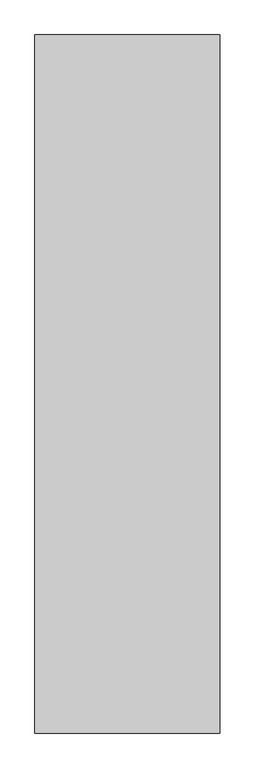
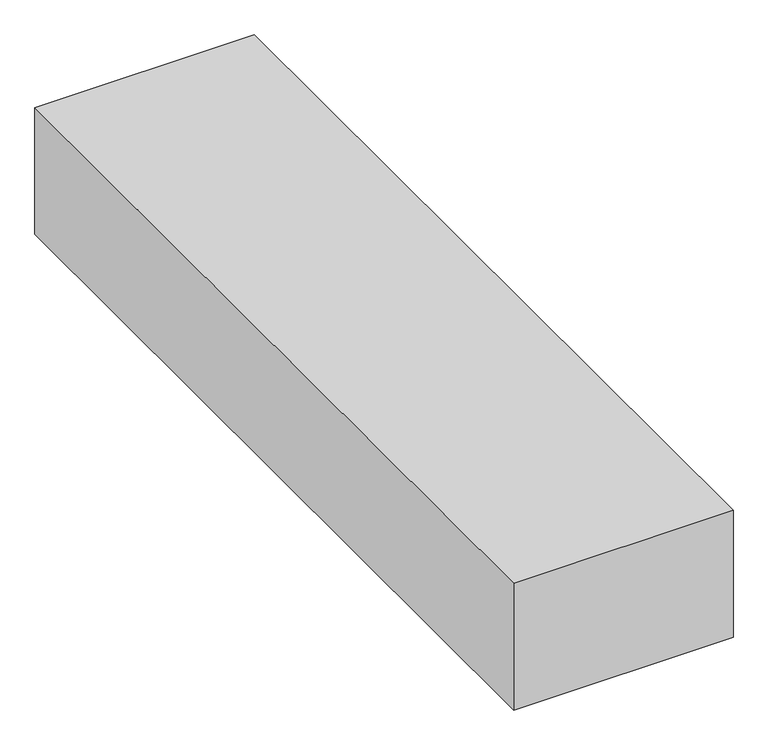
"""IFC4 building model written with IfcOpenShell, lengths in millimetres: proxy geometry, Space Planning Box_hec : Space Planning Box_hec."""

import ifcopenshell
import ifcopenshell.guid

model = None  # the IFC model being written
_history = None  # IfcOwnerHistory: only IFC2X3 demands one
_inside = {}  # id of a spatial element -> (the spatial element, [elements in it])
_under = {}  # id of a project, library or spatial element -> (it, [spatial elements below it])
_declared = {}  # id of a project -> (the project, [libraries it declares])
_typed = {}  # id of a type object -> (the type object, [elements of that type])
_made_of = {}  # id of a material, layer set ... -> (it, [elements and type objects made of it])


def new_model(schema):
    """Start an empty IFC model of exactly this schema.

    Asked for "IFC4X3", IfcOpenShell would pick the latest addendum, in which some entities
    have other attributes; the version numbers below select the first issue.
    IFC2X3 requires an IfcOwnerHistory on every rooted entity: one is made here for all.
    """
    global model, _history
    if schema == "IFC4X3":
        model = ifcopenshell.file(schema_version=(4, 3, 0, 0))
    else:
        model = ifcopenshell.file(schema=schema)
    _inside.clear()
    _under.clear()
    _declared.clear()
    _typed.clear()
    _made_of.clear()
    _history = None
    if model.schema == "IFC2X3":
        org = make("IfcOrganization", Name="unknown")
        user = make(
            "IfcPersonAndOrganization",
            ThePerson=make("IfcPerson", FamilyName="unknown"),
            TheOrganization=org,
        )
        app = make(
            "IfcApplication",
            ApplicationDeveloper=org,
            Version="unknown",
            ApplicationFullName="unknown",
            ApplicationIdentifier="unknown",
        )
        _history = make(
            "IfcOwnerHistory",
            OwningUser=user,
            OwningApplication=app,
            ChangeAction="ADDED",
            CreationDate=0,
        )
    return model


def make(cls, **values):
    """One entity of the class cls with the attributes given. An attribute that is None is left unset."""
    return model.create_entity(
        cls, **{name: value for name, value in values.items() if value is not None}
    )


def rooted(cls, **values):
    """An entity with a GlobalId (a new one), such as an element, a storey or a relation."""
    return make(cls, GlobalId=ifcopenshell.guid.new(), OwnerHistory=_history, **values)


def si_unit(unit_type, name, prefix=None):
    """IfcSIUnit, for example si_unit("LENGTHUNIT", "METRE", prefix="MILLI")."""
    return make("IfcSIUnit", UnitType=unit_type, Prefix=prefix, Name=name)


def assignment(units):
    """IfcUnitAssignment: the units of a project."""
    return None if units is None else make("IfcUnitAssignment", Units=units)


def point(xyz):
    """IfcCartesianPoint."""
    return None if xyz is None else make("IfcCartesianPoint", Coordinates=xyz)


def direction(xyz):
    """IfcDirection."""
    return None if xyz is None else make("IfcDirection", DirectionRatios=xyz)


def frame(location, z_axis=None, x_axis=None):
    """IfcAxis2Placement3D, a coordinate frame: its origin and axes. An axis left out is left unset."""
    return make(
        "IfcAxis2Placement3D",
        Location=point(location),
        Axis=direction(z_axis),
        RefDirection=direction(x_axis),
    )


def origin():
    """The frame at (0, 0, 0) with its axes left unset."""
    return frame((0.0, 0.0, 0.0))


def origin_with_axes():
    """The frame at (0, 0, 0) with the z axis (0, 0, 1) and the x axis (1, 0, 0) written out."""
    return frame((0.0, 0.0, 0.0), z_axis=(0.0, 0.0, 1.0), x_axis=(1.0, 0.0, 0.0))


def place(relative_to, where):
    """IfcLocalPlacement: puts the frame where relative to a parent placement (None: the world)."""
    return make(
        "IfcLocalPlacement", PlacementRelTo=relative_to, RelativePlacement=where
    )


def context(
    kind, dimensions, precision=None, world=None, true_north=None, identifier=None
):
    """IfcGeometricRepresentationContext, for example the 3D "Model" context."""
    return make(
        "IfcGeometricRepresentationContext",
        ContextIdentifier=identifier,
        ContextType=kind,
        CoordinateSpaceDimension=dimensions,
        Precision=precision,
        WorldCoordinateSystem=world,
        TrueNorth=true_north,
    )


def project(units=None, contexts=None):
    """IfcProject with its units and contexts."""
    return rooted(
        "IfcProject",
        Name="project",
        RepresentationContexts=contexts,
        UnitsInContext=assignment(units),
    )


def spatial(cls, under=None, at=None, **own):
    """A site, building, storey or space (cls), placed at a placement, below another one or the project."""
    s = rooted(cls, ObjectPlacement=at, **own)
    if under is not None:
        _under.setdefault(under.id(), (under, []))[1].append(s)
    return s


def polyline(points):
    """IfcPolyline through the points."""
    return make("IfcPolyline", Points=[point(p) for p in points])


def outline(outer, holes=None, kind="AREA"):
    """IfcArbitraryClosedProfileDef: a profile drawn as a closed curve; with holes, ...WithVoids."""
    if holes is None:
        return make("IfcArbitraryClosedProfileDef", ProfileType=kind, OuterCurve=outer)
    return make(
        "IfcArbitraryProfileDefWithVoids",
        ProfileType=kind,
        OuterCurve=outer,
        InnerCurves=holes,
    )


def extrude(swept, where, along, depth):
    """IfcExtrudedAreaSolid: the profile swept, set in the frame where, extruded along a direction by depth."""
    return make(
        "IfcExtrudedAreaSolid",
        SweptArea=swept,
        Position=where,
        ExtrudedDirection=direction(along),
        Depth=depth,
    )


def shape(context_of_items, identifier, shape_type, items):
    """IfcShapeRepresentation: the items that make up one representation, for example the "Body"."""
    return make(
        "IfcShapeRepresentation",
        ContextOfItems=context_of_items,
        RepresentationIdentifier=identifier,
        RepresentationType=shape_type,
        Items=items,
    )


def source(mapping_origin, context_of_items, identifier, shape_type, items):
    """IfcRepresentationMap: a shape defined once, which mapped items show again and again."""
    return make(
        "IfcRepresentationMap",
        MappingOrigin=mapping_origin,
        MappedRepresentation=shape(context_of_items, identifier, shape_type, items),
    )


def transform(
    local_origin,
    x_axis=None,
    y_axis=None,
    z_axis=None,
    scale=None,
    scale2=None,
    scale3=None,
    uniform=True,
):
    """IfcCartesianTransformationOperator3D, or its non-uniform kind. x_axis, y_axis, z_axis: its Axis1, 2, 3."""
    if uniform:
        return make(
            "IfcCartesianTransformationOperator3D",
            Axis1=direction(x_axis),
            Axis2=direction(y_axis),
            LocalOrigin=point(local_origin),
            Scale=scale,
            Axis3=direction(z_axis),
        )
    return make(
        "IfcCartesianTransformationOperator3DnonUniform",
        Axis1=direction(x_axis),
        Axis2=direction(y_axis),
        LocalOrigin=point(local_origin),
        Scale=scale,
        Axis3=direction(z_axis),
        Scale2=scale2,
        Scale3=scale3,
    )


def mapped(mapping_source, mapping_target):
    """IfcMappedItem: shows the shape of a source again, moved by a transform."""
    return make(
        "IfcMappedItem", MappingSource=mapping_source, MappingTarget=mapping_target
    )


def made_of(thing, what):
    """Note that an element or type object is made of a material, layer set ...; save() writes the relation."""
    if what is not None:
        _made_of.setdefault(what.id(), (what, []))[1].append(thing)
    return thing


def element(
    cls,
    number,
    at=None,
    inside=None,
    cuts=None,
    type_object=None,
    material=None,
    context=None,
    identifier="Body",
    shape_type=None,
    held_by="IfcProductDefinitionShape",
    body=None,
    shapes=None,
    **own,
):
    """One element of the class cls, such as IfcWall. Its Tag is "e" and its number.

    at: its placement. inside: the storey or other place that contains it. cuts: it is an
    opening in that element (IfcRelVoidsElement). A single representation is given by context,
    identifier, shape_type and body (its items); several are given by shapes. held_by: the class
    of the entity that holds the representations. save() writes the other relations.
    """
    e = rooted(cls, Tag="e%d" % number, ObjectPlacement=at, **own)
    if body is not None:
        shapes = [shape(context, identifier, shape_type, body)]
    if shapes is not None:
        e.Representation = make(held_by, Representations=shapes)
    if inside is not None:
        _inside.setdefault(inside.id(), (inside, []))[1].append(e)
    if cuts is not None:
        rooted(
            "IfcRelVoidsElement", RelatingBuildingElement=cuts, RelatedOpeningElement=e
        )
    if type_object is not None:
        _typed.setdefault(type_object.id(), (type_object, []))[1].append(e)
    return made_of(e, material)


def aggregate(whole, parts):
    """IfcRelAggregates: a whole, such as a stair, and the parts it consists of."""
    return rooted("IfcRelAggregates", RelatingObject=whole, RelatedObjects=parts)


def save(model, path):
    """Write the relations noted so far, then the file.

    IfcRelAggregates (storeys below a building ...), IfcRelContainedInSpatialStructure (elements
    in a storey), IfcRelDefinesByType, IfcRelAssociatesMaterial and IfcRelDeclares: one each for
    every whole, place, type object, material and project.
    """
    for whole, parts in _under.values():
        aggregate(whole, parts)
    for where, things in _inside.values():
        rooted(
            "IfcRelContainedInSpatialStructure",
            RelatedElements=things,
            RelatingStructure=where,
        )
    for kind, things in _typed.values():
        rooted("IfcRelDefinesByType", RelatedObjects=things, RelatingType=kind)
    for what, things in _made_of.values():
        rooted("IfcRelAssociatesMaterial", RelatedObjects=things, RelatingMaterial=what)
    for by, libraries in _declared.values():
        rooted("IfcRelDeclares", RelatingContext=by, RelatedDefinitions=libraries)
    model.write(path)


def generic_models_8b5775ea(model_context):
    return source(origin(), model_context, "Body", "SweptSolid", [
        extrude(outline(polyline([(4500.0, 17000.0), (4500.0, -17000.0), (-4500.0, -17000.0), (-4500.0, 17000.0), (4500.0, 17000.0)])), origin_with_axes(), (0.0, 0.0, 1.0), 5500.0),
    ])


if __name__ == "__main__":
    model = new_model("IFC4")
    model_context = context("Model", 3, world=origin())
    ifc_project = project(units=[si_unit("LENGTHUNIT", "METRE", prefix="MILLI")], contexts=[model_context])
    site = spatial("IfcSite", under=ifc_project)
    building = spatial("IfcBuilding", under=site)
    placement = place(None, origin())
    generic_models_shape = generic_models_8b5775ea(model_context)
    element("IfcBuildingElementProxy", 1, Name="Space Planning Box_hec : Space Planning Box_hec", ObjectType="Space Planning Box_hec : Space Planning Box_hec", at=placement, inside=building, context=model_context, shape_type="MappedRepresentation", body=[
        mapped(generic_models_shape, transform((0.0, 0.0, 0.0), x_axis=(1.0, 0.0, 0.0), y_axis=(0.0, 1.0, 0.0), z_axis=(0.0, 0.0, 1.0))),
    ])
    save(model, "model.ifc")

# Revit data of these elements
# Project information
#   Building Name = "MAIN GATE SECURITY BUILDING"
#   Project Status = "Project Status"
#   Client Name = "현대엔지니어링"
#   Project Address = "서울시 종로구 율곡로 75(계동)"
#   Project Name = "Therma Visayas Energy Project"
#   Project Number = "-"
# Type "Space Planning Box_hec : Space Planning Box_hec"
#   Type Comments = "..."
#   Room Name [instance default] = "?"
#   Interior Finish [instance default] = ""
#   Exterior Finish [instance default] = ""
#   Department [instance default] = ""
#   Assembly Code = "..."
#   Width [instance default] = 1524 mm
#   Program Area [instance default] = 0.00 m²
#   Length [instance default] = 1524 mm
#   Height [instance default] = 1524 mm
#   Area [instance default] = 2.32258 m²
#   Fill Color [instance default] = Cyan
#   Default Elevation = 0
# Element 1 (IfcBuildingElementProxy, "Space Planning Box_hec : Space Planning Box_hec")
#   Room Name = "Electrical Room-2"
#   Interior Finish = "IW5..N/A..N/A,,WK1..N/A,,FL1,,CL1..N/A"
#   Exterior Finish = "N/A..N/A,,EW1..EW2..N/A"
#   Department = "EL"
#   Width = 9000 mm
#   Program Area = 288.00 m²
#   Length = 34000 mm
#   Height = 5500 mm
#   Area = 306.00 m²
#   Fill Color = Orange
#   Materials on its faces: "Orange"
# Materials
#   "Cyan": class "Generic", colour RGB 0 255 255, transparency 0.2, Cost = 0
#   "Orange": class "Generic", colour RGB 255 165 0, transparency 0.2, Cost = 0
